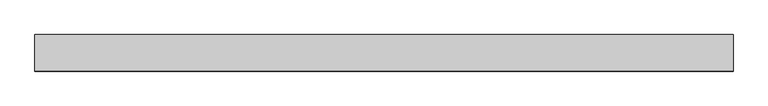
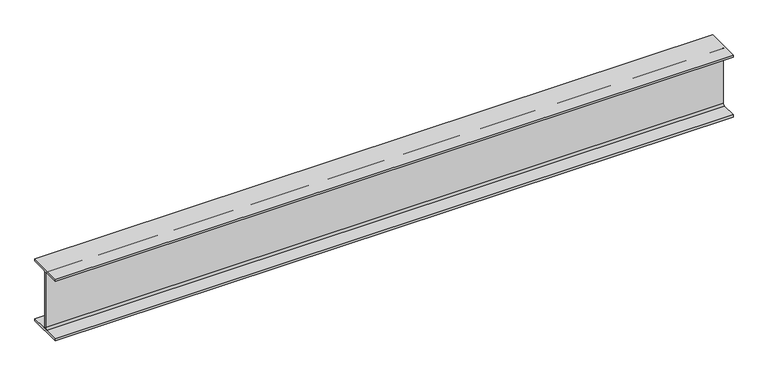
"""IFC4 building model written with IfcOpenShell, lengths in millimetres: beam geometry, Steel Beam_H-KSD3502 : H_SB_ASB_H-250x125x6x9."""

import ifcopenshell
import ifcopenshell.guid

model = None  # the IFC model being written
_history = None  # IfcOwnerHistory: only IFC2X3 demands one
_inside = {}  # id of a spatial element -> (the spatial element, [elements in it])
_under = {}  # id of a project, library or spatial element -> (it, [spatial elements below it])
_declared = {}  # id of a project -> (the project, [libraries it declares])
_typed = {}  # id of a type object -> (the type object, [elements of that type])
_made_of = {}  # id of a material, layer set ... -> (it, [elements and type objects made of it])


def new_model(schema):
    """Start an empty IFC model of exactly this schema.

    Asked for "IFC4X3", IfcOpenShell would pick the latest addendum, in which some entities
    have other attributes; the version numbers below select the first issue.
    IFC2X3 requires an IfcOwnerHistory on every rooted entity: one is made here for all.
    """
    global model, _history
    if schema == "IFC4X3":
        model = ifcopenshell.file(schema_version=(4, 3, 0, 0))
    else:
        model = ifcopenshell.file(schema=schema)
    _inside.clear()
    _under.clear()
    _declared.clear()
    _typed.clear()
    _made_of.clear()
    _history = None
    if model.schema == "IFC2X3":
        org = make("IfcOrganization", Name="unknown")
        user = make(
            "IfcPersonAndOrganization",
            ThePerson=make("IfcPerson", FamilyName="unknown"),
            TheOrganization=org,
        )
        app = make(
            "IfcApplication",
            ApplicationDeveloper=org,
            Version="unknown",
            ApplicationFullName="unknown",
            ApplicationIdentifier="unknown",
        )
        _history = make(
            "IfcOwnerHistory",
            OwningUser=user,
            OwningApplication=app,
            ChangeAction="ADDED",
            CreationDate=0,
        )
    return model


def make(cls, **values):
    """One entity of the class cls with the attributes given. An attribute that is None is left unset."""
    return model.create_entity(
        cls, **{name: value for name, value in values.items() if value is not None}
    )


def rooted(cls, **values):
    """An entity with a GlobalId (a new one), such as an element, a storey or a relation."""
    return make(cls, GlobalId=ifcopenshell.guid.new(), OwnerHistory=_history, **values)


def si_unit(unit_type, name, prefix=None):
    """IfcSIUnit, for example si_unit("LENGTHUNIT", "METRE", prefix="MILLI")."""
    return make("IfcSIUnit", UnitType=unit_type, Prefix=prefix, Name=name)


def assignment(units):
    """IfcUnitAssignment: the units of a project."""
    return None if units is None else make("IfcUnitAssignment", Units=units)


def point(xyz):
    """IfcCartesianPoint."""
    return None if xyz is None else make("IfcCartesianPoint", Coordinates=xyz)


def direction(xyz):
    """IfcDirection."""
    return None if xyz is None else make("IfcDirection", DirectionRatios=xyz)


def frame(location, z_axis=None, x_axis=None):
    """IfcAxis2Placement3D, a coordinate frame: its origin and axes. An axis left out is left unset."""
    return make(
        "IfcAxis2Placement3D",
        Location=point(location),
        Axis=direction(z_axis),
        RefDirection=direction(x_axis),
    )


def frame_2d(location, x_axis=None):
    """IfcAxis2Placement2D, a coordinate frame in the plane: its origin and x axis."""
    return make(
        "IfcAxis2Placement2D", Location=point(location), RefDirection=direction(x_axis)
    )


def origin():
    """The frame at (0, 0, 0) with its axes left unset."""
    return frame((0.0, 0.0, 0.0))


def place(relative_to, where):
    """IfcLocalPlacement: puts the frame where relative to a parent placement (None: the world)."""
    return make(
        "IfcLocalPlacement", PlacementRelTo=relative_to, RelativePlacement=where
    )


def context(
    kind, dimensions, precision=None, world=None, true_north=None, identifier=None
):
    """IfcGeometricRepresentationContext, for example the 3D "Model" context."""
    return make(
        "IfcGeometricRepresentationContext",
        ContextIdentifier=identifier,
        ContextType=kind,
        CoordinateSpaceDimension=dimensions,
        Precision=precision,
        WorldCoordinateSystem=world,
        TrueNorth=true_north,
    )


def project(units=None, contexts=None):
    """IfcProject with its units and contexts."""
    return rooted(
        "IfcProject",
        Name="project",
        RepresentationContexts=contexts,
        UnitsInContext=assignment(units),
    )


def spatial(cls, under=None, at=None, **own):
    """A site, building, storey or space (cls), placed at a placement, below another one or the project."""
    s = rooted(cls, ObjectPlacement=at, **own)
    if under is not None:
        _under.setdefault(under.id(), (under, []))[1].append(s)
    return s


def polyline(points):
    """IfcPolyline through the points."""
    return make("IfcPolyline", Points=[point(p) for p in points])


def circle_curve(where, radius):
    """IfcCircle in the frame where."""
    return make("IfcCircle", Position=where, Radius=radius)


def trimmed(basis, trim1, trim2, sense, master):
    """IfcTrimmedCurve: the piece of a basis curve between two trims."""
    return make(
        "IfcTrimmedCurve",
        BasisCurve=basis,
        Trim1=trim1,
        Trim2=trim2,
        SenseAgreement=sense,
        MasterRepresentation=master,
    )


def segment(curve, same_sense, transition):
    """IfcCompositeCurveSegment."""
    return make(
        "IfcCompositeCurveSegment",
        Transition=transition,
        SameSense=same_sense,
        ParentCurve=curve,
    )


def composite_curve(segments, self_intersect=None):
    """IfcCompositeCurve: segments joined end to end."""
    return make("IfcCompositeCurve", Segments=segments, SelfIntersect=self_intersect)


def outline(outer, holes=None, kind="AREA"):
    """IfcArbitraryClosedProfileDef: a profile drawn as a closed curve; with holes, ...WithVoids."""
    if holes is None:
        return make("IfcArbitraryClosedProfileDef", ProfileType=kind, OuterCurve=outer)
    return make(
        "IfcArbitraryProfileDefWithVoids",
        ProfileType=kind,
        OuterCurve=outer,
        InnerCurves=holes,
    )


def extrude(swept, where, along, depth):
    """IfcExtrudedAreaSolid: the profile swept, set in the frame where, extruded along a direction by depth."""
    return make(
        "IfcExtrudedAreaSolid",
        SweptArea=swept,
        Position=where,
        ExtrudedDirection=direction(along),
        Depth=depth,
    )


def shape(context_of_items, identifier, shape_type, items):
    """IfcShapeRepresentation: the items that make up one representation, for example the "Body"."""
    return make(
        "IfcShapeRepresentation",
        ContextOfItems=context_of_items,
        RepresentationIdentifier=identifier,
        RepresentationType=shape_type,
        Items=items,
    )


def source(mapping_origin, context_of_items, identifier, shape_type, items):
    """IfcRepresentationMap: a shape defined once, which mapped items show again and again."""
    return make(
        "IfcRepresentationMap",
        MappingOrigin=mapping_origin,
        MappedRepresentation=shape(context_of_items, identifier, shape_type, items),
    )


def transform(
    local_origin,
    x_axis=None,
    y_axis=None,
    z_axis=None,
    scale=None,
    scale2=None,
    scale3=None,
    uniform=True,
):
    """IfcCartesianTransformationOperator3D, or its non-uniform kind. x_axis, y_axis, z_axis: its Axis1, 2, 3."""
    if uniform:
        return make(
            "IfcCartesianTransformationOperator3D",
            Axis1=direction(x_axis),
            Axis2=direction(y_axis),
            LocalOrigin=point(local_origin),
            Scale=scale,
            Axis3=direction(z_axis),
        )
    return make(
        "IfcCartesianTransformationOperator3DnonUniform",
        Axis1=direction(x_axis),
        Axis2=direction(y_axis),
        LocalOrigin=point(local_origin),
        Scale=scale,
        Axis3=direction(z_axis),
        Scale2=scale2,
        Scale3=scale3,
    )


def mapped(mapping_source, mapping_target):
    """IfcMappedItem: shows the shape of a source again, moved by a transform."""
    return make(
        "IfcMappedItem", MappingSource=mapping_source, MappingTarget=mapping_target
    )


def made_of(thing, what):
    """Note that an element or type object is made of a material, layer set ...; save() writes the relation."""
    if what is not None:
        _made_of.setdefault(what.id(), (what, []))[1].append(thing)
    return thing


def element(
    cls,
    number,
    at=None,
    inside=None,
    cuts=None,
    type_object=None,
    material=None,
    context=None,
    identifier="Body",
    shape_type=None,
    held_by="IfcProductDefinitionShape",
    body=None,
    shapes=None,
    **own,
):
    """One element of the class cls, such as IfcWall. Its Tag is "e" and its number.

    at: its placement. inside: the storey or other place that contains it. cuts: it is an
    opening in that element (IfcRelVoidsElement). A single representation is given by context,
    identifier, shape_type and body (its items); several are given by shapes. held_by: the class
    of the entity that holds the representations. save() writes the other relations.
    """
    e = rooted(cls, Tag="e%d" % number, ObjectPlacement=at, **own)
    if body is not None:
        shapes = [shape(context, identifier, shape_type, body)]
    if shapes is not None:
        e.Representation = make(held_by, Representations=shapes)
    if inside is not None:
        _inside.setdefault(inside.id(), (inside, []))[1].append(e)
    if cuts is not None:
        rooted(
            "IfcRelVoidsElement", RelatingBuildingElement=cuts, RelatedOpeningElement=e
        )
    if type_object is not None:
        _typed.setdefault(type_object.id(), (type_object, []))[1].append(e)
    return made_of(e, material)


def aggregate(whole, parts):
    """IfcRelAggregates: a whole, such as a stair, and the parts it consists of."""
    return rooted("IfcRelAggregates", RelatingObject=whole, RelatedObjects=parts)


def save(model, path):
    """Write the relations noted so far, then the file.

    IfcRelAggregates (storeys below a building ...), IfcRelContainedInSpatialStructure (elements
    in a storey), IfcRelDefinesByType, IfcRelAssociatesMaterial and IfcRelDeclares: one each for
    every whole, place, type object, material and project.
    """
    for whole, parts in _under.values():
        aggregate(whole, parts)
    for where, things in _inside.values():
        rooted(
            "IfcRelContainedInSpatialStructure",
            RelatedElements=things,
            RelatingStructure=where,
        )
    for kind, things in _typed.values():
        rooted("IfcRelDefinesByType", RelatedObjects=things, RelatingType=kind)
    for what, things in _made_of.values():
        rooted("IfcRelAssociatesMaterial", RelatedObjects=things, RelatingMaterial=what)
    for by, libraries in _declared.values():
        rooted("IfcRelDeclares", RelatingContext=by, RelatedDefinitions=libraries)
    model.write(path)


def beam_1b59f9ff(model_context):
    return source(origin(), model_context, "Body", "SweptSolid", [
        extrude(outline(composite_curve([segment(polyline([(82.5, -141.5), (82.5, -151.7), (-82.5, -151.7), (-82.5, -141.5), (-11.9, -141.5)]), True, "CONTINUOUS"), segment(trimmed(circle_curve(frame_2d((-11.9, -132.6)), 8.9), [point((-11.9, -141.5))], [point((-3.0, -132.6))], True, "CARTESIAN"), True, "CONTINUOUS"), segment(polyline([(-3.0, -132.6), (-3.0, 132.6)]), True, "CONTINUOUS"), segment(trimmed(circle_curve(frame_2d((-11.9, 132.6)), 8.9), [point((-3.0, 132.6))], [point((-11.9, 141.5))], True, "CARTESIAN"), True, "CONTINUOUS"), segment(polyline([(-11.9, 141.5), (-82.5, 141.5), (-82.5, 151.7), (82.5, 151.7), (82.5, 141.5), (11.9, 141.5)]), True, "CONTINUOUS"), segment(trimmed(circle_curve(frame_2d((11.9, 132.6)), 8.9), [point((11.9, 141.5))], [point((3.0, 132.6))], True, "CARTESIAN"), True, "CONTINUOUS"), segment(polyline([(3.0, 132.6), (3.0, -132.6)]), True, "CONTINUOUS"), segment(trimmed(circle_curve(frame_2d((11.9, -132.6)), 8.9), [point((3.0, -132.6))], [point((11.9, -141.5))], True, "CARTESIAN"), True, "CONTINUOUS"), segment(polyline([(11.9, -141.5), (82.5, -141.5)]), True, "CONTINUOUS")], self_intersect=False)), frame((-1494.4889476, 0.0, 0.0), z_axis=(1.0, 0.0, 0.0), x_axis=(0.0, 1.0, 0.0)), (0.0, 0.0, 1.0), 3149.288991),
    ])


if __name__ == "__main__":
    model = new_model("IFC4")
    model_context = context("Model", 3, world=origin())
    ifc_project = project(units=[si_unit("LENGTHUNIT", "METRE", prefix="MILLI")], contexts=[model_context])
    site = spatial("IfcSite", under=ifc_project)
    building = spatial("IfcBuilding", under=site)
    placement = place(None, origin())
    beam_shape = beam_1b59f9ff(model_context)
    element("IfcBeam", 1, ObjectType="Steel Beam_H-KSD3502 : H_SB_ASB_H-250x125x6x9", at=placement, inside=building, context=model_context, shape_type="MappedRepresentation", body=[
        mapped(beam_shape, transform((0.0, 0.0, 0.0), x_axis=(1.0, 0.0, 0.0), y_axis=(0.0, 1.0, 0.0), z_axis=(0.0, 0.0, 1.0))),
    ])
    save(model, "model.ifc")

# Revit data of these elements
# Type "Steel Beam_H-KSD3502 : H_SB_ASB_H-250x125x6x9"
#   Width = 12.5 cm
#   Web Thickness = 0.6 cm
#   Web Fillet = 1.2 cm
#   Warping Constant = 42539.8 cm⁶
#   Torsional Moment of Inertia = 7.8102 cm⁴
#   Torsional Modulus = 1.0 cm³
#   Section Area = 37.66 cm²
#   Plastic Modulus weak axis = 73.1 cm³
#   Plastic Modulus strong axis = 366.0 cm³
#   Perimeter = 0.97 m²/m
#   Nominal Weight = 29.60 kgf/m
#   Moment of Inertia weak axis = 294.00 cm⁴
#   Moment of Inertia strong axis = 4050.00 cm⁴
#   Height = 25.0 cm
#   Flange Thickness = 0.9 cm
#   Elastic Modulus weak axis = 47.0 cm³
#   Elastic Modulus strong axis = 324.0 cm³
#   Centroid Vertical = 12.5 cm
#   Centroid Horizontal = 6.25 cm
#   Length [instance default] = 1.5240 m
#   Structural Material [instance default] = Steel, 45-345
#   Assembly Code = ""
# Element 1 (IfcBeam, "Steel Beam_H-KSD3502 : H_SB_ASB_H-250x125x6x9")
#   Structural Material = none
# Materials
#   "Steel, 45-345": class "Metal", colour RGB 189 187 185, transparency 0, Description = "Steel 345 MPa", Cost = 0
